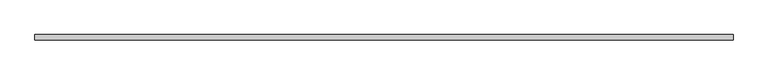
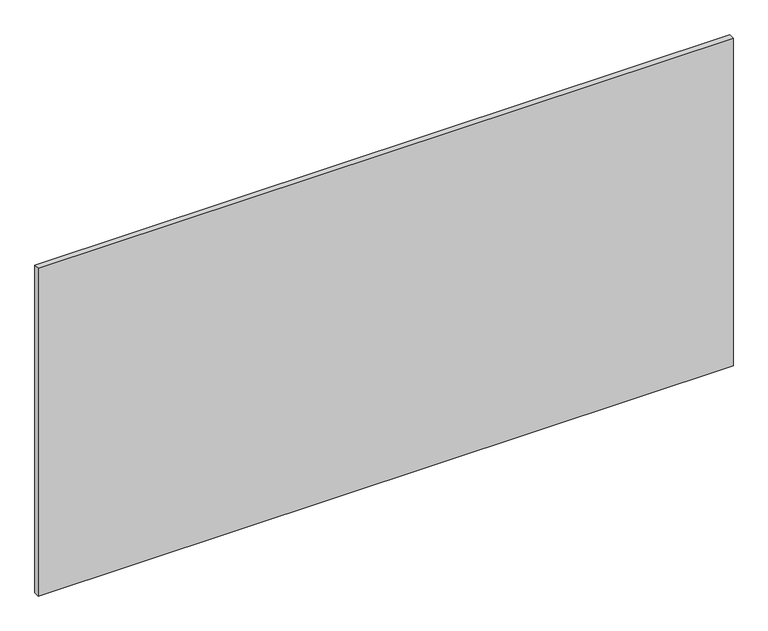
"""IFC4 building model written with IfcOpenShell, lengths in millimetres: proxy geometry, Inner panel:Inner panel:1:Inner panel:1 : Inner panel:Inner panel:300324:300043:Inner panel:1:Inner panel:1 : Inner panel:Inner panel:300324:300043 : Inner panel:Inner panel:1:Inner panel:1 : Inner panel:Inner panel:300324:300043:1 : Inner panel:Inner panel:1:Inner panel:1 : Inner panel:Inner panel:300324:300043:Inner panel:1:Inner panel:1 : Inner panel:Inner panel:300324:300043 : Inner panel:Inner panel:1:Inner panel:1 : Inner panel:Inner panel:300324:300043:300031."""

import ifcopenshell
import ifcopenshell.guid

model = None  # the IFC model being written
_history = None  # IfcOwnerHistory: only IFC2X3 demands one
_inside = {}  # id of a spatial element -> (the spatial element, [elements in it])
_under = {}  # id of a project, library or spatial element -> (it, [spatial elements below it])
_declared = {}  # id of a project -> (the project, [libraries it declares])
_typed = {}  # id of a type object -> (the type object, [elements of that type])
_made_of = {}  # id of a material, layer set ... -> (it, [elements and type objects made of it])


def new_model(schema):
    """Start an empty IFC model of exactly this schema.

    Asked for "IFC4X3", IfcOpenShell would pick the latest addendum, in which some entities
    have other attributes; the version numbers below select the first issue.
    IFC2X3 requires an IfcOwnerHistory on every rooted entity: one is made here for all.
    """
    global model, _history
    if schema == "IFC4X3":
        model = ifcopenshell.file(schema_version=(4, 3, 0, 0))
    else:
        model = ifcopenshell.file(schema=schema)
    _inside.clear()
    _under.clear()
    _declared.clear()
    _typed.clear()
    _made_of.clear()
    _history = None
    if model.schema == "IFC2X3":
        org = make("IfcOrganization", Name="unknown")
        user = make(
            "IfcPersonAndOrganization",
            ThePerson=make("IfcPerson", FamilyName="unknown"),
            TheOrganization=org,
        )
        app = make(
            "IfcApplication",
            ApplicationDeveloper=org,
            Version="unknown",
            ApplicationFullName="unknown",
            ApplicationIdentifier="unknown",
        )
        _history = make(
            "IfcOwnerHistory",
            OwningUser=user,
            OwningApplication=app,
            ChangeAction="ADDED",
            CreationDate=0,
        )
    return model


def make(cls, **values):
    """One entity of the class cls with the attributes given. An attribute that is None is left unset."""
    return model.create_entity(
        cls, **{name: value for name, value in values.items() if value is not None}
    )


def rooted(cls, **values):
    """An entity with a GlobalId (a new one), such as an element, a storey or a relation."""
    return make(cls, GlobalId=ifcopenshell.guid.new(), OwnerHistory=_history, **values)


def si_unit(unit_type, name, prefix=None):
    """IfcSIUnit, for example si_unit("LENGTHUNIT", "METRE", prefix="MILLI")."""
    return make("IfcSIUnit", UnitType=unit_type, Prefix=prefix, Name=name)


def assignment(units):
    """IfcUnitAssignment: the units of a project."""
    return None if units is None else make("IfcUnitAssignment", Units=units)


def point(xyz):
    """IfcCartesianPoint."""
    return None if xyz is None else make("IfcCartesianPoint", Coordinates=xyz)


def direction(xyz):
    """IfcDirection."""
    return None if xyz is None else make("IfcDirection", DirectionRatios=xyz)


def frame(location, z_axis=None, x_axis=None):
    """IfcAxis2Placement3D, a coordinate frame: its origin and axes. An axis left out is left unset."""
    return make(
        "IfcAxis2Placement3D",
        Location=point(location),
        Axis=direction(z_axis),
        RefDirection=direction(x_axis),
    )


def origin():
    """The frame at (0, 0, 0) with its axes left unset."""
    return frame((0.0, 0.0, 0.0))


def place(relative_to, where):
    """IfcLocalPlacement: puts the frame where relative to a parent placement (None: the world)."""
    return make(
        "IfcLocalPlacement", PlacementRelTo=relative_to, RelativePlacement=where
    )


def context(
    kind, dimensions, precision=None, world=None, true_north=None, identifier=None
):
    """IfcGeometricRepresentationContext, for example the 3D "Model" context."""
    return make(
        "IfcGeometricRepresentationContext",
        ContextIdentifier=identifier,
        ContextType=kind,
        CoordinateSpaceDimension=dimensions,
        Precision=precision,
        WorldCoordinateSystem=world,
        TrueNorth=true_north,
    )


def project(units=None, contexts=None):
    """IfcProject with its units and contexts."""
    return rooted(
        "IfcProject",
        Name="project",
        RepresentationContexts=contexts,
        UnitsInContext=assignment(units),
    )


def spatial(cls, under=None, at=None, **own):
    """A site, building, storey or space (cls), placed at a placement, below another one or the project."""
    s = rooted(cls, ObjectPlacement=at, **own)
    if under is not None:
        _under.setdefault(under.id(), (under, []))[1].append(s)
    return s


def polyline(points):
    """IfcPolyline through the points."""
    return make("IfcPolyline", Points=[point(p) for p in points])


def outline(outer, holes=None, kind="AREA"):
    """IfcArbitraryClosedProfileDef: a profile drawn as a closed curve; with holes, ...WithVoids."""
    if holes is None:
        return make("IfcArbitraryClosedProfileDef", ProfileType=kind, OuterCurve=outer)
    return make(
        "IfcArbitraryProfileDefWithVoids",
        ProfileType=kind,
        OuterCurve=outer,
        InnerCurves=holes,
    )


def extrude(swept, where, along, depth):
    """IfcExtrudedAreaSolid: the profile swept, set in the frame where, extruded along a direction by depth."""
    return make(
        "IfcExtrudedAreaSolid",
        SweptArea=swept,
        Position=where,
        ExtrudedDirection=direction(along),
        Depth=depth,
    )


def shape(context_of_items, identifier, shape_type, items):
    """IfcShapeRepresentation: the items that make up one representation, for example the "Body"."""
    return make(
        "IfcShapeRepresentation",
        ContextOfItems=context_of_items,
        RepresentationIdentifier=identifier,
        RepresentationType=shape_type,
        Items=items,
    )


def source(mapping_origin, context_of_items, identifier, shape_type, items):
    """IfcRepresentationMap: a shape defined once, which mapped items show again and again."""
    return make(
        "IfcRepresentationMap",
        MappingOrigin=mapping_origin,
        MappedRepresentation=shape(context_of_items, identifier, shape_type, items),
    )


def transform(
    local_origin,
    x_axis=None,
    y_axis=None,
    z_axis=None,
    scale=None,
    scale2=None,
    scale3=None,
    uniform=True,
):
    """IfcCartesianTransformationOperator3D, or its non-uniform kind. x_axis, y_axis, z_axis: its Axis1, 2, 3."""
    if uniform:
        return make(
            "IfcCartesianTransformationOperator3D",
            Axis1=direction(x_axis),
            Axis2=direction(y_axis),
            LocalOrigin=point(local_origin),
            Scale=scale,
            Axis3=direction(z_axis),
        )
    return make(
        "IfcCartesianTransformationOperator3DnonUniform",
        Axis1=direction(x_axis),
        Axis2=direction(y_axis),
        LocalOrigin=point(local_origin),
        Scale=scale,
        Axis3=direction(z_axis),
        Scale2=scale2,
        Scale3=scale3,
    )


def mapped(mapping_source, mapping_target):
    """IfcMappedItem: shows the shape of a source again, moved by a transform."""
    return make(
        "IfcMappedItem", MappingSource=mapping_source, MappingTarget=mapping_target
    )


def made_of(thing, what):
    """Note that an element or type object is made of a material, layer set ...; save() writes the relation."""
    if what is not None:
        _made_of.setdefault(what.id(), (what, []))[1].append(thing)
    return thing


def element(
    cls,
    number,
    at=None,
    inside=None,
    cuts=None,
    type_object=None,
    material=None,
    context=None,
    identifier="Body",
    shape_type=None,
    held_by="IfcProductDefinitionShape",
    body=None,
    shapes=None,
    **own,
):
    """One element of the class cls, such as IfcWall. Its Tag is "e" and its number.

    at: its placement. inside: the storey or other place that contains it. cuts: it is an
    opening in that element (IfcRelVoidsElement). A single representation is given by context,
    identifier, shape_type and body (its items); several are given by shapes. held_by: the class
    of the entity that holds the representations. save() writes the other relations.
    """
    e = rooted(cls, Tag="e%d" % number, ObjectPlacement=at, **own)
    if body is not None:
        shapes = [shape(context, identifier, shape_type, body)]
    if shapes is not None:
        e.Representation = make(held_by, Representations=shapes)
    if inside is not None:
        _inside.setdefault(inside.id(), (inside, []))[1].append(e)
    if cuts is not None:
        rooted(
            "IfcRelVoidsElement", RelatingBuildingElement=cuts, RelatedOpeningElement=e
        )
    if type_object is not None:
        _typed.setdefault(type_object.id(), (type_object, []))[1].append(e)
    return made_of(e, material)


def aggregate(whole, parts):
    """IfcRelAggregates: a whole, such as a stair, and the parts it consists of."""
    return rooted("IfcRelAggregates", RelatingObject=whole, RelatedObjects=parts)


def save(model, path):
    """Write the relations noted so far, then the file.

    IfcRelAggregates (storeys below a building ...), IfcRelContainedInSpatialStructure (elements
    in a storey), IfcRelDefinesByType, IfcRelAssociatesMaterial and IfcRelDeclares: one each for
    every whole, place, type object, material and project.
    """
    for whole, parts in _under.values():
        aggregate(whole, parts)
    for where, things in _inside.values():
        rooted(
            "IfcRelContainedInSpatialStructure",
            RelatedElements=things,
            RelatingStructure=where,
        )
    for kind, things in _typed.values():
        rooted("IfcRelDefinesByType", RelatedObjects=things, RelatingType=kind)
    for what, things in _made_of.values():
        rooted("IfcRelAssociatesMaterial", RelatedObjects=things, RelatingMaterial=what)
    for by, libraries in _declared.values():
        rooted("IfcRelDeclares", RelatingContext=by, RelatedDefinitions=libraries)
    model.write(path)


def generic_models_14970219(model_context):
    return source(origin(), model_context, "Body", "SweptSolid", [
        extrude(outline(polyline([(593738.0867239, -578778.4413841), (596182.8367239, -578778.4413841), (596182.8367239, -578797.4913841), (593738.0867239, -578797.4913841), (593738.0867239, -578778.4413841)])), frame((0.0, 0.0, 44.45), z_axis=(0.0, 0.0, 1.0), x_axis=(1.0, 0.0, 0.0)), (0.0, 0.0, 1.0), 1219.2),
    ])


if __name__ == "__main__":
    model = new_model("IFC4")
    model_context = context("Model", 3, world=origin())
    ifc_project = project(units=[si_unit("LENGTHUNIT", "METRE", prefix="MILLI")], contexts=[model_context])
    site = spatial("IfcSite", under=ifc_project)
    building = spatial("IfcBuilding", under=site)
    placement = place(None, origin())
    generic_models_shape = generic_models_14970219(model_context)
    element("IfcBuildingElementProxy", 1, Name="Inner panel:Inner panel:1:Inner panel:1 : Inner panel:Inner panel:300324:300043:Inner panel:1:Inner panel:1 : Inner panel:Inner panel:300324:300043 : Inner panel:Inner panel:1:Inner panel:1 : Inner panel:Inner panel:300324:300043:1 : Inner panel:Inner panel:1:Inner panel:1 : Inner panel:Inner panel:300324:300043:Inner panel:1:Inner panel:1 : Inner panel:Inner panel:300324:300043 : Inner panel:Inner panel:1:Inner panel:1 : Inner panel:Inner panel:300324:300043:300031", ObjectType="Inner panel:Inner panel:1:Inner panel:1 : Inner panel:Inner panel:300324:300043:Inner panel:1:Inner panel:1 : Inner panel:Inner panel:300324:300043 : Inner panel:Inner panel:1:Inner panel:1 : Inner panel:Inner panel:300324:300043:1 : Inner panel:Inner panel:1:Inner panel:1 : Inner panel:Inner panel:300324:300043:Inner panel:1:Inner panel:1 : Inner panel:Inner panel:300324:300043 : Inner panel:Inner panel:1:Inner panel:1 : Inner panel:Inner panel:300324:300043:300031", at=placement, inside=building, context=model_context, shape_type="MappedRepresentation", body=[
        mapped(generic_models_shape, transform((0.0, 0.0, 0.0), x_axis=(1.0, 0.0, 0.0), y_axis=(0.0, 1.0, 0.0), z_axis=(0.0, 0.0, 1.0))),
    ])
    save(model, "model.ifc")

# Revit data of these elements
# Type "Inner panel:Inner panel:1:Inner panel:1 : Inner panel:Inner panel:300324:300043:Inner panel:1:Inner panel:1 : Inner panel:Inner panel:300324:300043 : Inner panel:Inner panel:1:Inner panel:1 : Inner panel:Inner panel:300324:300043:1 : Inner panel:Inner panel:1:Inner panel:1 : Inner panel:Inner panel:300324:300043:Inner panel:1:Inner panel:1 : Inner panel:Inner panel:300324:300043 : Inner panel:Inner panel:1:Inner panel:1 : Inner panel:Inner panel:300324:300043:300031"
#   NameOverride = "Inner panel:Inner panel:1:Inner panel:1 : Inner panel:Inner panel:300324:300043:Inner panel:1:Inner panel:1 : Inner panel:Inner panel:300324:300043 : Inner panel:Inner panel:1:Inner panel:1 : Inner panel:Inner panel:300324:300043:300031"
#   ObjectTypeOverride = "Inner panel:1:Inner panel:1 : Inner panel:Inner panel:300324:300043 : Inner panel:Inner panel:1:Inner panel:1 : Inner panel:Inner panel:300324:300043"
#   Reference = "Inner panel"
#   Tag = "300031"
# Element 1 (IfcBuildingElementProxy, "Inner panel:Inner panel:1:Inner panel:1 : Inner panel:Inner panel:300324:300043:Inner panel:1:Inner panel:1 : Inner panel:Inner panel:300324:300043 : Inner panel:Inner panel:1:Inner panel:1 : Inner panel:Inner panel:300324:300043:1 : Inner panel:Inner panel:1:Inner panel:1 : Inner panel:Inner panel:300324:300043:Inner panel:1:Inner panel:1 : Inner panel:Inner panel:300324:300043 : Inner panel:Inner panel:1:Inner panel:1 : Inner panel:Inner panel:300324:300043:300031")
#   Materials on its faces: "¾” (CLASS A) FIRE RETARDANT PLYWOOD ...OR… IF 1/4\" GYP. BD UNDER PLYWOOD, FLAME SPREAD TO BE CLASS C -  (FINISH: GRADE B - PREFINISHED STAINED/SEALED) - 1/4\" GAP BTWN PANELS (FASTENERS T.B.D.)"
# Materials
#   "¾” (CLASS A) FIRE RETARDANT PLYWOOD ...OR… IF 1/4\" GYP. BD UNDER PLYWOOD, FLAME SPREAD TO BE CLASS C -  (FINISH: GRADE B - PREFINISHED STAINED/SEALED) - 1/4\" GAP BTWN PANELS (FASTENERS T.B.D.)": class "Wood", colour RGB 149 120 74, transparency 0, Description = "Plywood, sheathing grade", Cost = 0
